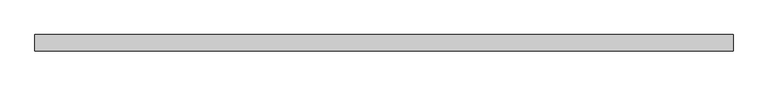
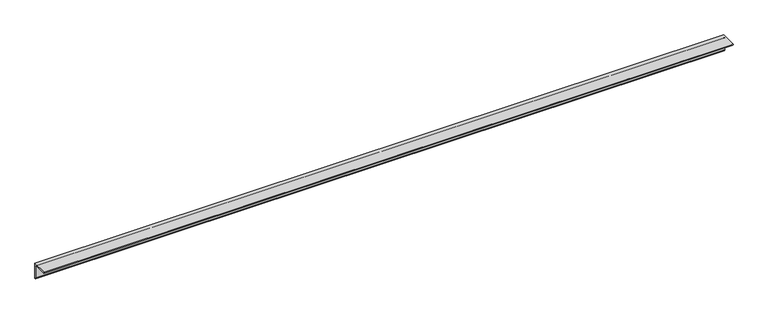
"""IFC4 building model written with IfcOpenShell, lengths in millimetres: member geometry, 0912_Steel Framing_L-KSD3502 : H_SB_AR_S03_L-130x130x12_HBR3."""

from ifc_helpers import new_model, si_unit, point, frame, frame_2d, origin, place, context, project, spatial, polyline, circle_curve, trimmed, segment, composite_curve, outline, extrude, source, transform, mapped, element, save


def member_53cbeec2(model_context):
    return source(origin(), model_context, "Body", "SweptSolid", [
        extrude(outline(composite_curve([segment(polyline([(36.4, 36.4), (36.4, -93.6)]), True, "CONTINUOUS"), segment(trimmed(circle_curve(frame_2d((36.4, -81.6)), 12.0), [point((36.4, -93.6))], [point((24.4, -81.6))], False, "CARTESIAN"), True, "CONTINUOUS"), segment(polyline([(24.4, -81.6), (24.4, 12.4)]), True, "CONTINUOUS"), segment(trimmed(circle_curve(frame_2d((12.4, 12.4)), 12.0), [point((24.4, 12.4))], [point((12.4, 24.4))], True, "CARTESIAN"), True, "CONTINUOUS"), segment(polyline([(12.4, 24.4), (-81.6, 24.4)]), True, "CONTINUOUS"), segment(trimmed(circle_curve(frame_2d((-81.6, 36.4)), 12.0), [point((-81.6, 24.4))], [point((-93.6, 36.4))], False, "CARTESIAN"), True, "CONTINUOUS"), segment(polyline([(-93.6, 36.4), (36.4, 36.4)]), True, "CONTINUOUS")], self_intersect=False)), frame((-2753.7999994, 0.0, 0.0), z_axis=(1.0, 0.0, 0.0), x_axis=(0.0, 1.0, 0.0)), (0.0, 0.0, 1.0), 5507.5999988),
    ])


if __name__ == "__main__":
    model = new_model("IFC4")
    model_context = context("Model", 3, world=origin())
    ifc_project = project(units=[si_unit("LENGTHUNIT", "METRE", prefix="MILLI")], contexts=[model_context])
    site = spatial("IfcSite", under=ifc_project)
    building = spatial("IfcBuilding", under=site)
    placement = place(None, origin())
    member_shape = member_53cbeec2(model_context)
    element("IfcMember", 1, ObjectType="0912_Steel Framing_L-KSD3502 : H_SB_AR_S03_L-130x130x12_HBR3", at=placement, inside=building, context=model_context, shape_type="MappedRepresentation", body=[
        mapped(member_shape, transform((0.0, 0.0, 0.0), x_axis=(1.0, 0.0, 0.0), y_axis=(0.0, 1.0, 0.0), z_axis=(0.0, 0.0, 1.0))),
    ])
    save(model, "model.ifc")

# Revit data of these elements
# Type "0912_Steel Framing_L-KSD3502 : H_SB_AR_S03_L-130x130x12_HBR3"
#   k = 25 mm
#   Perimeter = 0.52 m²/m
#   Nominal Weight = 23.40 kgf/m
#   Length [instance default] = 1000 mm
#   b = 130 mm
#   d = 130 mm
#   t = 12 mm
#   x = 36.4 mm
#   y = 36.4 mm
#   A = 2976.00 m²
#   Structural Material [instance default] = Steel, 45-345
# Element 1 (IfcMember, "0912_Steel Framing_L-KSD3502 : H_SB_AR_S03_L-130x130x12_HBR3")
#   Materials on its faces: "Steel, 45-345"
# Materials
#   "Steel, 45-345": class "Metal", colour RGB 189 187 185, transparency 0, Description = "Steel 345 MPa", Cost = 0
